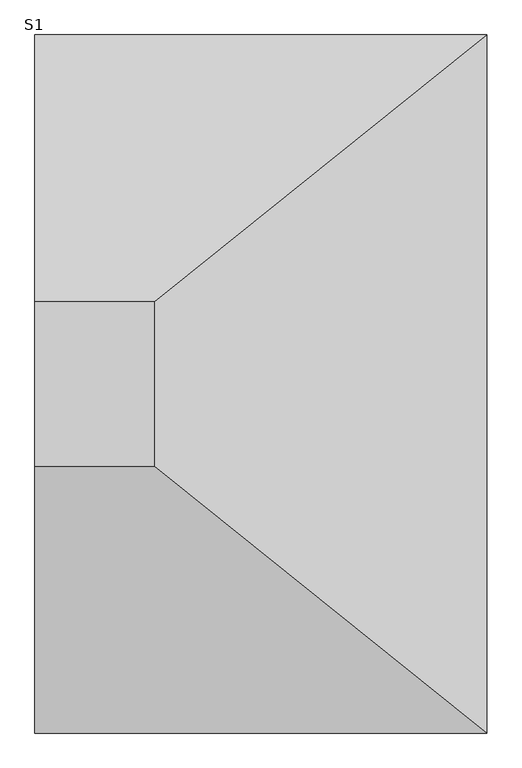
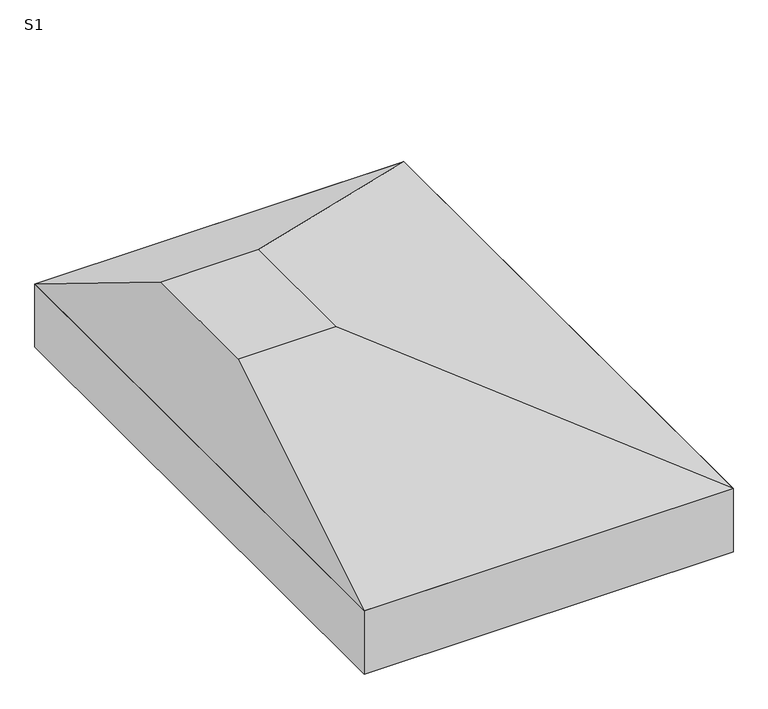
"""IFC4 building model written with IfcOpenShell, lengths in millimetres: fastener geometry, TQS - Sapata : S1."""

import ifcopenshell
import ifcopenshell.guid

model = None  # the IFC model being written
_history = None  # IfcOwnerHistory: only IFC2X3 demands one
_inside = {}  # id of a spatial element -> (the spatial element, [elements in it])
_under = {}  # id of a project, library or spatial element -> (it, [spatial elements below it])
_declared = {}  # id of a project -> (the project, [libraries it declares])
_typed = {}  # id of a type object -> (the type object, [elements of that type])
_made_of = {}  # id of a material, layer set ... -> (it, [elements and type objects made of it])


def new_model(schema):
    """Start an empty IFC model of exactly this schema.

    Asked for "IFC4X3", IfcOpenShell would pick the latest addendum, in which some entities
    have other attributes; the version numbers below select the first issue.
    IFC2X3 requires an IfcOwnerHistory on every rooted entity: one is made here for all.
    """
    global model, _history
    if schema == "IFC4X3":
        model = ifcopenshell.file(schema_version=(4, 3, 0, 0))
    else:
        model = ifcopenshell.file(schema=schema)
    _inside.clear()
    _under.clear()
    _declared.clear()
    _typed.clear()
    _made_of.clear()
    _history = None
    if model.schema == "IFC2X3":
        org = make("IfcOrganization", Name="unknown")
        user = make(
            "IfcPersonAndOrganization",
            ThePerson=make("IfcPerson", FamilyName="unknown"),
            TheOrganization=org,
        )
        app = make(
            "IfcApplication",
            ApplicationDeveloper=org,
            Version="unknown",
            ApplicationFullName="unknown",
            ApplicationIdentifier="unknown",
        )
        _history = make(
            "IfcOwnerHistory",
            OwningUser=user,
            OwningApplication=app,
            ChangeAction="ADDED",
            CreationDate=0,
        )
    return model


def make(cls, **values):
    """One entity of the class cls with the attributes given. An attribute that is None is left unset."""
    return model.create_entity(
        cls, **{name: value for name, value in values.items() if value is not None}
    )


def rooted(cls, **values):
    """An entity with a GlobalId (a new one), such as an element, a storey or a relation."""
    return make(cls, GlobalId=ifcopenshell.guid.new(), OwnerHistory=_history, **values)


def si_unit(unit_type, name, prefix=None):
    """IfcSIUnit, for example si_unit("LENGTHUNIT", "METRE", prefix="MILLI")."""
    return make("IfcSIUnit", UnitType=unit_type, Prefix=prefix, Name=name)


def assignment(units):
    """IfcUnitAssignment: the units of a project."""
    return None if units is None else make("IfcUnitAssignment", Units=units)


def point(xyz):
    """IfcCartesianPoint."""
    return None if xyz is None else make("IfcCartesianPoint", Coordinates=xyz)


def direction(xyz):
    """IfcDirection."""
    return None if xyz is None else make("IfcDirection", DirectionRatios=xyz)


def frame(location, z_axis=None, x_axis=None):
    """IfcAxis2Placement3D, a coordinate frame: its origin and axes. An axis left out is left unset."""
    return make(
        "IfcAxis2Placement3D",
        Location=point(location),
        Axis=direction(z_axis),
        RefDirection=direction(x_axis),
    )


def origin():
    """The frame at (0, 0, 0) with its axes left unset."""
    return frame((0.0, 0.0, 0.0))


def place(relative_to, where):
    """IfcLocalPlacement: puts the frame where relative to a parent placement (None: the world)."""
    return make(
        "IfcLocalPlacement", PlacementRelTo=relative_to, RelativePlacement=where
    )


def context(
    kind, dimensions, precision=None, world=None, true_north=None, identifier=None
):
    """IfcGeometricRepresentationContext, for example the 3D "Model" context."""
    return make(
        "IfcGeometricRepresentationContext",
        ContextIdentifier=identifier,
        ContextType=kind,
        CoordinateSpaceDimension=dimensions,
        Precision=precision,
        WorldCoordinateSystem=world,
        TrueNorth=true_north,
    )


def project(units=None, contexts=None):
    """IfcProject with its units and contexts."""
    return rooted(
        "IfcProject",
        Name="project",
        RepresentationContexts=contexts,
        UnitsInContext=assignment(units),
    )


def spatial(cls, under=None, at=None, **own):
    """A site, building, storey or space (cls), placed at a placement, below another one or the project."""
    s = rooted(cls, ObjectPlacement=at, **own)
    if under is not None:
        _under.setdefault(under.id(), (under, []))[1].append(s)
    return s


def polyline(points):
    """IfcPolyline through the points."""
    return make("IfcPolyline", Points=[point(p) for p in points])


def outline(outer, holes=None, kind="AREA"):
    """IfcArbitraryClosedProfileDef: a profile drawn as a closed curve; with holes, ...WithVoids."""
    if holes is None:
        return make("IfcArbitraryClosedProfileDef", ProfileType=kind, OuterCurve=outer)
    return make(
        "IfcArbitraryProfileDefWithVoids",
        ProfileType=kind,
        OuterCurve=outer,
        InnerCurves=holes,
    )


def extrude(swept, where, along, depth):
    """IfcExtrudedAreaSolid: the profile swept, set in the frame where, extruded along a direction by depth."""
    return make(
        "IfcExtrudedAreaSolid",
        SweptArea=swept,
        Position=where,
        ExtrudedDirection=direction(along),
        Depth=depth,
    )


def faces_of(points, faces, orient=None, outer=None):
    """IfcFace entities. A face is a list of loops; a loop is a list of indices into points, from 0.

    orient and outer hold one flag for each loop. By default every Orientation is true, the
    first loop of a face is its IfcFaceOuterBound and the others are IfcFaceBound.
    """
    made = []
    for i, loops in enumerate(faces):
        bounds = []
        for j, loop in enumerate(loops):
            is_outer = j == 0 if outer is None else outer[i][j]
            bounds.append(
                make(
                    "IfcFaceOuterBound" if is_outer else "IfcFaceBound",
                    Bound=make("IfcPolyLoop", Polygon=[points[k] for k in loop]),
                    Orientation=True if orient is None else orient[i][j],
                )
            )
        made.append(make("IfcFace", Bounds=bounds))
    return made


def faceted_brep(points, faces, orient=None, outer=None, voids=None):
    """IfcFacetedBrep: a solid bounded by flat faces; with voids (closed shells), ...WithVoids."""
    shared = [point(p) for p in points]
    hull = make("IfcClosedShell", CfsFaces=faces_of(shared, faces, orient, outer))
    if voids is None:
        return make("IfcFacetedBrep", Outer=hull)
    return make(
        "IfcFacetedBrepWithVoids",
        Outer=hull,
        Voids=[
            make(cls, CfsFaces=faces_of(shared, fs, o, b)) for cls, fs, o, b in voids
        ],
    )


def shape(context_of_items, identifier, shape_type, items):
    """IfcShapeRepresentation: the items that make up one representation, for example the "Body"."""
    return make(
        "IfcShapeRepresentation",
        ContextOfItems=context_of_items,
        RepresentationIdentifier=identifier,
        RepresentationType=shape_type,
        Items=items,
    )


def source(mapping_origin, context_of_items, identifier, shape_type, items):
    """IfcRepresentationMap: a shape defined once, which mapped items show again and again."""
    return make(
        "IfcRepresentationMap",
        MappingOrigin=mapping_origin,
        MappedRepresentation=shape(context_of_items, identifier, shape_type, items),
    )


def transform(
    local_origin,
    x_axis=None,
    y_axis=None,
    z_axis=None,
    scale=None,
    scale2=None,
    scale3=None,
    uniform=True,
):
    """IfcCartesianTransformationOperator3D, or its non-uniform kind. x_axis, y_axis, z_axis: its Axis1, 2, 3."""
    if uniform:
        return make(
            "IfcCartesianTransformationOperator3D",
            Axis1=direction(x_axis),
            Axis2=direction(y_axis),
            LocalOrigin=point(local_origin),
            Scale=scale,
            Axis3=direction(z_axis),
        )
    return make(
        "IfcCartesianTransformationOperator3DnonUniform",
        Axis1=direction(x_axis),
        Axis2=direction(y_axis),
        LocalOrigin=point(local_origin),
        Scale=scale,
        Axis3=direction(z_axis),
        Scale2=scale2,
        Scale3=scale3,
    )


def mapped(mapping_source, mapping_target):
    """IfcMappedItem: shows the shape of a source again, moved by a transform."""
    return make(
        "IfcMappedItem", MappingSource=mapping_source, MappingTarget=mapping_target
    )


def made_of(thing, what):
    """Note that an element or type object is made of a material, layer set ...; save() writes the relation."""
    if what is not None:
        _made_of.setdefault(what.id(), (what, []))[1].append(thing)
    return thing


def element(
    cls,
    number,
    at=None,
    inside=None,
    cuts=None,
    type_object=None,
    material=None,
    context=None,
    identifier="Body",
    shape_type=None,
    held_by="IfcProductDefinitionShape",
    body=None,
    shapes=None,
    **own,
):
    """One element of the class cls, such as IfcWall. Its Tag is "e" and its number.

    at: its placement. inside: the storey or other place that contains it. cuts: it is an
    opening in that element (IfcRelVoidsElement). A single representation is given by context,
    identifier, shape_type and body (its items); several are given by shapes. held_by: the class
    of the entity that holds the representations. save() writes the other relations.
    """
    e = rooted(cls, Tag="e%d" % number, ObjectPlacement=at, **own)
    if body is not None:
        shapes = [shape(context, identifier, shape_type, body)]
    if shapes is not None:
        e.Representation = make(held_by, Representations=shapes)
    if inside is not None:
        _inside.setdefault(inside.id(), (inside, []))[1].append(e)
    if cuts is not None:
        rooted(
            "IfcRelVoidsElement", RelatingBuildingElement=cuts, RelatedOpeningElement=e
        )
    if type_object is not None:
        _typed.setdefault(type_object.id(), (type_object, []))[1].append(e)
    return made_of(e, material)


def aggregate(whole, parts):
    """IfcRelAggregates: a whole, such as a stair, and the parts it consists of."""
    return rooted("IfcRelAggregates", RelatingObject=whole, RelatedObjects=parts)


def save(model, path):
    """Write the relations noted so far, then the file.

    IfcRelAggregates (storeys below a building ...), IfcRelContainedInSpatialStructure (elements
    in a storey), IfcRelDefinesByType, IfcRelAssociatesMaterial and IfcRelDeclares: one each for
    every whole, place, type object, material and project.
    """
    for whole, parts in _under.values():
        aggregate(whole, parts)
    for where, things in _inside.values():
        rooted(
            "IfcRelContainedInSpatialStructure",
            RelatedElements=things,
            RelatingStructure=where,
        )
    for kind, things in _typed.values():
        rooted("IfcRelDefinesByType", RelatedObjects=things, RelatingType=kind)
    for what, things in _made_of.values():
        rooted("IfcRelAssociatesMaterial", RelatedObjects=things, RelatingMaterial=what)
    for by, libraries in _declared.values():
        rooted("IfcRelDeclares", RelatingContext=by, RelatedDefinitions=libraries)
    model.write(path)


def s1_ccae0304(model_context):
    return source(origin(), model_context, "Body", "SolidModel", [
        faceted_brep([(-460.0, 0.0, 0.0), (-750.0, 0.0, 0.0), (-750.0, -400.0, 0.0), (-460.0, -400.0, 0.0), (350.0, 650.0, -400.0), (350.0, -1050.0, -400.0), (-750.0, -1050.0, -400.0), (-750.0, 650.0, -400.0)], [[[0, 1, 2, 3]], [[4, 5, 6, 7]], [[4, 7, 1, 0]], [[7, 6, 2, 1]], [[6, 5, 3, 2]], [[5, 4, 0, 3]]]),
        extrude(outline(polyline([(350.0, 650.0), (350.0, -1050.0), (-750.0, -1050.0), (-750.0, 650.0), (350.0, 650.0)])), frame((0.0, 0.0, -600.0), z_axis=(0.0, 0.0, 1.0), x_axis=(1.0, 0.0, 0.0)), (0.0, 0.0, 1.0), 200.0),
    ])


if __name__ == "__main__":
    model = new_model("IFC4")
    model_context = context("Model", 3, world=origin())
    ifc_project = project(units=[si_unit("LENGTHUNIT", "METRE", prefix="MILLI")], contexts=[model_context])
    site = spatial("IfcSite", under=ifc_project)
    building = spatial("IfcBuilding", under=site)
    placement = place(None, origin())
    s1_shape = s1_ccae0304(model_context)
    element("IfcFastener", 1, ObjectType="TQS - Sapata : S1", at=placement, inside=building, context=model_context, shape_type="MappedRepresentation", body=[
        mapped(s1_shape, transform((0.0, 0.0, 0.0), x_axis=(1.0, 0.0, 0.0), y_axis=(0.0, 1.0, 0.0), z_axis=(0.0, 0.0, 1.0))),
    ])
    save(model, "model.ifc")

# Revit data of these elements
# Type "TQS - Sapata : S1"
#   TY = 0.40 m
#   TX = 0.29 m
#   HS = 0.60 m
#   H0 = 0.20 m
#   EXCYABS = 0.85 m
#   EXCY = 0.00 m
#   EXCXABS = 0.145 m
#   EXCX = -0.405 m
#   DIMY = 1.70 m
#   DIMX = 1.10 m
#   Material estrutural = Concreto - Concreto concretado no local
#   Width = 0
#   Length = 0
# Element 1 (IfcFastener, "TQS - Sapata : S1")
#   Materials on its faces: "Concreto - Concreto concretado no local"
# Materials
#   "Concreto - Concreto concretado no local": class "Concreto", colour RGB 192 192 192, transparency 0
